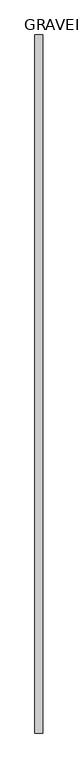
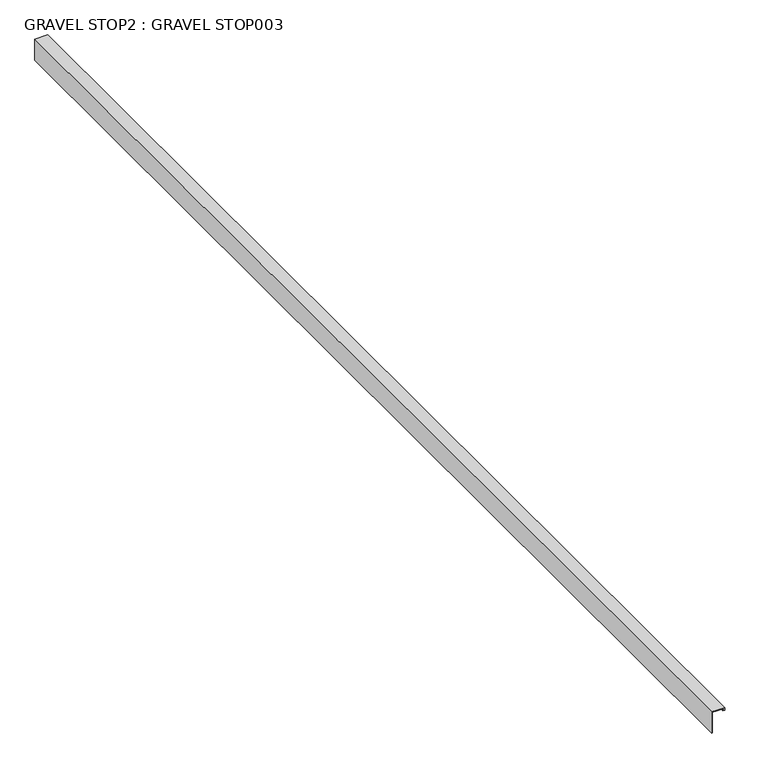
"""IFC4 building model written with IfcOpenShell, lengths in millimetres: proxy geometry, GRAVEL STOP2 : GRAVEL STOP003."""

from ifc_helpers import new_model, si_unit, frame, origin, place, context, project, spatial, polyline, outline, extrude, source, transform, mapped, element, save


def gravel_stop2_gravel_stop003_5ef83285(model_context):
    return source(origin(), model_context, "Body", "SweptSolid", [
        extrude(outline(polyline([(40234.4061757, -4378.3539248), (40234.4061757, -4358.6689248), (40232.1963757, -4358.6689248), (40232.1963757, -4360.4013812), (40230.9263757, -4360.4013812), (40230.9263757, -4357.3989248), (40235.6761757, -4357.3989248), (40235.6761757, -4379.6239248), (40197.5761757, -4379.6239248), (40197.5761757, -4378.3539248), (40234.4061757, -4378.3539248)])), frame((0.0, -1052.8906573, 0.0), z_axis=(0.0, 1.0, 0.0), x_axis=(0.0, 0.0, 1.0)), (0.0, 0.0, 1.0), 2000.25),
    ])


if __name__ == "__main__":
    model = new_model("IFC4")
    model_context = context("Model", 3, world=origin())
    ifc_project = project(units=[si_unit("LENGTHUNIT", "METRE", prefix="MILLI")], contexts=[model_context])
    site = spatial("IfcSite", under=ifc_project)
    building = spatial("IfcBuilding", under=site)
    placement = place(None, origin())
    gravel_stop2_gravel_stop003_shape = gravel_stop2_gravel_stop003_5ef83285(model_context)
    element("IfcBuildingElementProxy", 1, Name="GRAVEL STOP2 : GRAVEL STOP003", ObjectType="GRAVEL STOP2 : GRAVEL STOP003", at=placement, inside=building, context=model_context, shape_type="MappedRepresentation", body=[
        mapped(gravel_stop2_gravel_stop003_shape, transform((0.0, 0.0, 0.0), x_axis=(1.0, 0.0, 0.0), y_axis=(0.0, 1.0, 0.0), z_axis=(0.0, 0.0, 1.0))),
    ])
    save(model, "model.ifc")

# Revit data of these elements
# Type "GRAVEL STOP2 : GRAVEL STOP003"
#   NameOverride = "GRAVEL STOP003"
# Element 1 (IfcBuildingElementProxy, "GRAVEL STOP2 : GRAVEL STOP003")
#   Materials on its faces: "COPPER STUCCO J BEAD"
# Materials
#   "COPPER STUCCO J BEAD": class "Unassigned", colour RGB 251 232 155, transparency 0, Cost = 0
